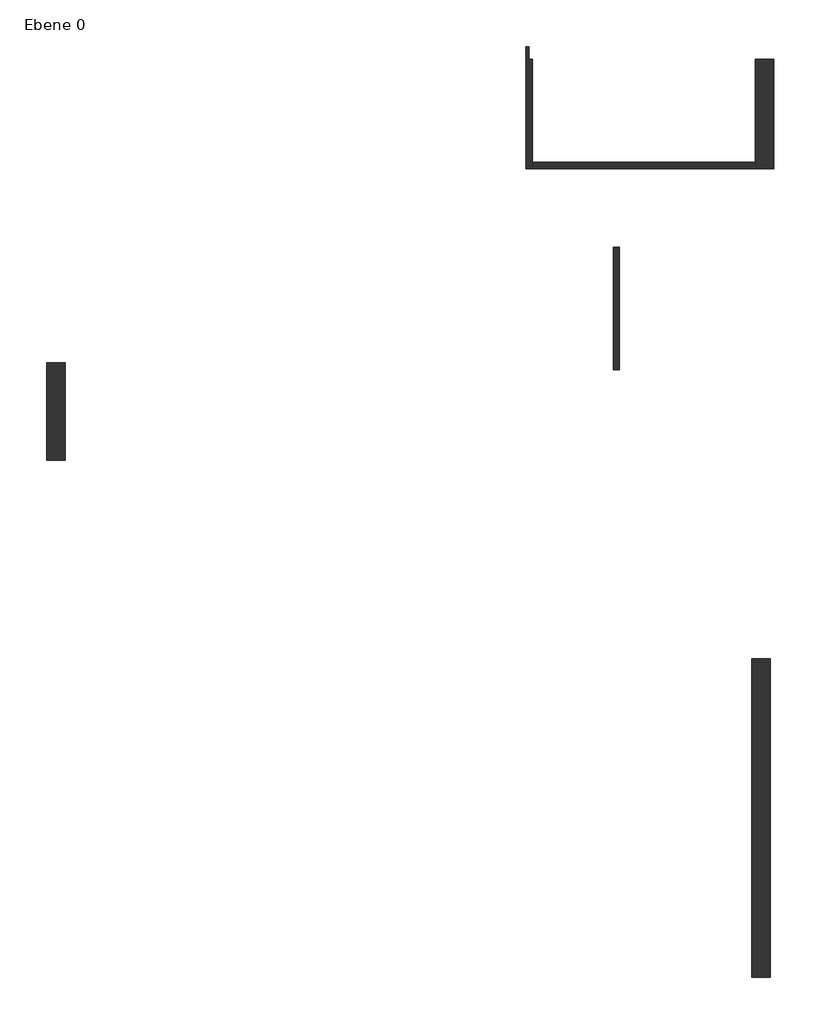
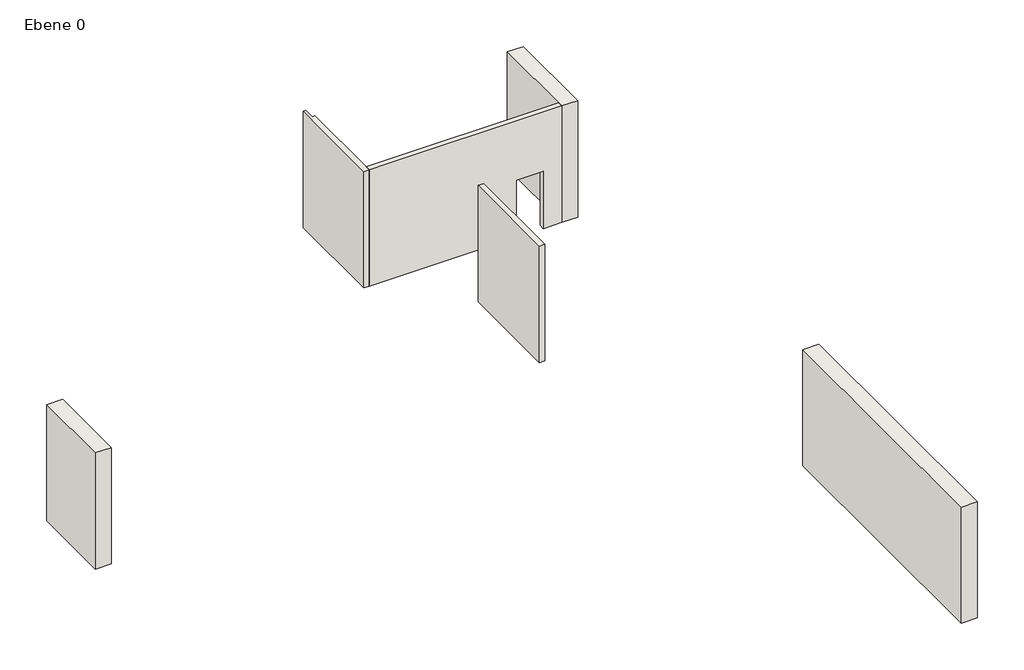
# One storey: 6 walls.
"""IFC4 building model written with IfcOpenShell, lengths in millimetres."""

import ifcopenshell
import ifcopenshell.guid

model = None  # the IFC model being written
_history = None  # IfcOwnerHistory: only IFC2X3 demands one
_inside = {}  # id of a spatial element -> (the spatial element, [elements in it])
_under = {}  # id of a project, library or spatial element -> (it, [spatial elements below it])
_declared = {}  # id of a project -> (the project, [libraries it declares])
_typed = {}  # id of a type object -> (the type object, [elements of that type])
_made_of = {}  # id of a material, layer set ... -> (it, [elements and type objects made of it])


def new_model(schema):
    """Start an empty IFC model of exactly this schema.

    Asked for "IFC4X3", IfcOpenShell would pick the latest addendum, in which some entities
    have other attributes; the version numbers below select the first issue.
    IFC2X3 requires an IfcOwnerHistory on every rooted entity: one is made here for all.
    """
    global model, _history
    if schema == "IFC4X3":
        model = ifcopenshell.file(schema_version=(4, 3, 0, 0))
    else:
        model = ifcopenshell.file(schema=schema)
    _inside.clear()
    _under.clear()
    _declared.clear()
    _typed.clear()
    _made_of.clear()
    _history = None
    if model.schema == "IFC2X3":
        org = make("IfcOrganization", Name="unknown")
        user = make(
            "IfcPersonAndOrganization",
            ThePerson=make("IfcPerson", FamilyName="unknown"),
            TheOrganization=org,
        )
        app = make(
            "IfcApplication",
            ApplicationDeveloper=org,
            Version="unknown",
            ApplicationFullName="unknown",
            ApplicationIdentifier="unknown",
        )
        _history = make(
            "IfcOwnerHistory",
            OwningUser=user,
            OwningApplication=app,
            ChangeAction="ADDED",
            CreationDate=0,
        )
    return model


def make(cls, **values):
    """One entity of the class cls with the attributes given. An attribute that is None is left unset."""
    return model.create_entity(
        cls, **{name: value for name, value in values.items() if value is not None}
    )


def rooted(cls, **values):
    """An entity with a GlobalId (a new one), such as an element, a storey or a relation."""
    return make(cls, GlobalId=ifcopenshell.guid.new(), OwnerHistory=_history, **values)


def si_unit(unit_type, name, prefix=None):
    """IfcSIUnit, for example si_unit("LENGTHUNIT", "METRE", prefix="MILLI")."""
    return make("IfcSIUnit", UnitType=unit_type, Prefix=prefix, Name=name)


def assignment(units):
    """IfcUnitAssignment: the units of a project."""
    return None if units is None else make("IfcUnitAssignment", Units=units)


def point(xyz):
    """IfcCartesianPoint."""
    return None if xyz is None else make("IfcCartesianPoint", Coordinates=xyz)


def direction(xyz):
    """IfcDirection."""
    return None if xyz is None else make("IfcDirection", DirectionRatios=xyz)


def frame(location, z_axis=None, x_axis=None):
    """IfcAxis2Placement3D, a coordinate frame: its origin and axes. An axis left out is left unset."""
    return make(
        "IfcAxis2Placement3D",
        Location=point(location),
        Axis=direction(z_axis),
        RefDirection=direction(x_axis),
    )


def origin():
    """The frame at (0, 0, 0) with its axes left unset."""
    return frame((0.0, 0.0, 0.0))


def place(relative_to, where):
    """IfcLocalPlacement: puts the frame where relative to a parent placement (None: the world)."""
    return make(
        "IfcLocalPlacement", PlacementRelTo=relative_to, RelativePlacement=where
    )


def context(
    kind, dimensions, precision=None, world=None, true_north=None, identifier=None
):
    """IfcGeometricRepresentationContext, for example the 3D "Model" context."""
    return make(
        "IfcGeometricRepresentationContext",
        ContextIdentifier=identifier,
        ContextType=kind,
        CoordinateSpaceDimension=dimensions,
        Precision=precision,
        WorldCoordinateSystem=world,
        TrueNorth=true_north,
    )


def project(units=None, contexts=None):
    """IfcProject with its units and contexts."""
    return rooted(
        "IfcProject",
        Name="project",
        RepresentationContexts=contexts,
        UnitsInContext=assignment(units),
    )


def spatial(cls, under=None, at=None, **own):
    """A site, building, storey or space (cls), placed at a placement, below another one or the project."""
    s = rooted(cls, ObjectPlacement=at, **own)
    if under is not None:
        _under.setdefault(under.id(), (under, []))[1].append(s)
    return s


def polyline(points):
    """IfcPolyline through the points."""
    return make("IfcPolyline", Points=[point(p) for p in points])


def outline(outer, holes=None, kind="AREA"):
    """IfcArbitraryClosedProfileDef: a profile drawn as a closed curve; with holes, ...WithVoids."""
    if holes is None:
        return make("IfcArbitraryClosedProfileDef", ProfileType=kind, OuterCurve=outer)
    return make(
        "IfcArbitraryProfileDefWithVoids",
        ProfileType=kind,
        OuterCurve=outer,
        InnerCurves=holes,
    )


def extrude(swept, where, along, depth):
    """IfcExtrudedAreaSolid: the profile swept, set in the frame where, extruded along a direction by depth."""
    return make(
        "IfcExtrudedAreaSolid",
        SweptArea=swept,
        Position=where,
        ExtrudedDirection=direction(along),
        Depth=depth,
    )


def faces_of(points, faces, orient=None, outer=None):
    """IfcFace entities. A face is a list of loops; a loop is a list of indices into points, from 0.

    orient and outer hold one flag for each loop. By default every Orientation is true, the
    first loop of a face is its IfcFaceOuterBound and the others are IfcFaceBound.
    """
    made = []
    for i, loops in enumerate(faces):
        bounds = []
        for j, loop in enumerate(loops):
            is_outer = j == 0 if outer is None else outer[i][j]
            bounds.append(
                make(
                    "IfcFaceOuterBound" if is_outer else "IfcFaceBound",
                    Bound=make("IfcPolyLoop", Polygon=[points[k] for k in loop]),
                    Orientation=True if orient is None else orient[i][j],
                )
            )
        made.append(make("IfcFace", Bounds=bounds))
    return made


def faceted_brep(points, faces, orient=None, outer=None, voids=None):
    """IfcFacetedBrep: a solid bounded by flat faces; with voids (closed shells), ...WithVoids."""
    shared = [point(p) for p in points]
    hull = make("IfcClosedShell", CfsFaces=faces_of(shared, faces, orient, outer))
    if voids is None:
        return make("IfcFacetedBrep", Outer=hull)
    return make(
        "IfcFacetedBrepWithVoids",
        Outer=hull,
        Voids=[
            make(cls, CfsFaces=faces_of(shared, fs, o, b)) for cls, fs, o, b in voids
        ],
    )


def shape(context_of_items, identifier, shape_type, items):
    """IfcShapeRepresentation: the items that make up one representation, for example the "Body"."""
    return make(
        "IfcShapeRepresentation",
        ContextOfItems=context_of_items,
        RepresentationIdentifier=identifier,
        RepresentationType=shape_type,
        Items=items,
    )


def made_of(thing, what):
    """Note that an element or type object is made of a material, layer set ...; save() writes the relation."""
    if what is not None:
        _made_of.setdefault(what.id(), (what, []))[1].append(thing)
    return thing


def element(
    cls,
    number,
    at=None,
    inside=None,
    cuts=None,
    type_object=None,
    material=None,
    context=None,
    identifier="Body",
    shape_type=None,
    held_by="IfcProductDefinitionShape",
    body=None,
    shapes=None,
    **own,
):
    """One element of the class cls, such as IfcWall. Its Tag is "e" and its number.

    at: its placement. inside: the storey or other place that contains it. cuts: it is an
    opening in that element (IfcRelVoidsElement). A single representation is given by context,
    identifier, shape_type and body (its items); several are given by shapes. held_by: the class
    of the entity that holds the representations. save() writes the other relations.
    """
    e = rooted(cls, Tag="e%d" % number, ObjectPlacement=at, **own)
    if body is not None:
        shapes = [shape(context, identifier, shape_type, body)]
    if shapes is not None:
        e.Representation = make(held_by, Representations=shapes)
    if inside is not None:
        _inside.setdefault(inside.id(), (inside, []))[1].append(e)
    if cuts is not None:
        rooted(
            "IfcRelVoidsElement", RelatingBuildingElement=cuts, RelatedOpeningElement=e
        )
    if type_object is not None:
        _typed.setdefault(type_object.id(), (type_object, []))[1].append(e)
    return made_of(e, material)


def aggregate(whole, parts):
    """IfcRelAggregates: a whole, such as a stair, and the parts it consists of."""
    return rooted("IfcRelAggregates", RelatingObject=whole, RelatedObjects=parts)


def save(model, path):
    """Write the relations noted so far, then the file.

    IfcRelAggregates (storeys below a building ...), IfcRelContainedInSpatialStructure (elements
    in a storey), IfcRelDefinesByType, IfcRelAssociatesMaterial and IfcRelDeclares: one each for
    every whole, place, type object, material and project.
    """
    for whole, parts in _under.values():
        aggregate(whole, parts)
    for where, things in _inside.values():
        rooted(
            "IfcRelContainedInSpatialStructure",
            RelatedElements=things,
            RelatingStructure=where,
        )
    for kind, things in _typed.values():
        rooted("IfcRelDefinesByType", RelatedObjects=things, RelatingType=kind)
    for what, things in _made_of.values():
        rooted("IfcRelAssociatesMaterial", RelatedObjects=things, RelatingMaterial=what)
    for by, libraries in _declared.values():
        rooted("IfcRelDeclares", RelatingContext=by, RelatedDefinitions=libraries)
    model.write(path)


model = new_model("IFC4")

# Units and contexts
model_context = context("Model", 3, world=origin())
ifc_project = project(units=[si_unit("LENGTHUNIT", "METRE", prefix="MILLI")], contexts=[model_context])

# Site, building, storey
site = spatial("IfcSite", under=ifc_project)
building = spatial("IfcBuilding", under=site)
storey = spatial("IfcBuildingStorey", under=building, Name="Ebene 0", Elevation=0.0)

# Walls
placement = place(None, origin())
element("IfcWall", 1, ObjectType="STB 20.0", at=placement, inside=storey, context=model_context, shape_type="Brep", body=[
    faceted_brep([(5655.3173257, 15397.2389222, -1570.0), (5655.3173257, 11462.2122385, -1570.0), (5655.3173257, 11462.2122385, 3030.0), (5655.3173257, 15397.2389222, 3030.0), (5855.3173257, 14985.0055214, -1570.0), (5855.3173257, 14985.0055214, 3030.0), (5855.3173257, 11662.2122385, 3030.0), (5855.3173257, 11462.2122385, 3030.0), (5855.3173257, 11462.2122385, -1570.0), (5855.3173257, 11662.2122385, -1570.0), (5755.3173257, 15397.2389222, -1570.0), (5755.3173257, 14985.0055214, -1570.0), (5755.3173257, 14985.0055214, 3030.0), (5755.3173257, 15397.2389222, 3030.0)], [[[0, 1, 2, 3]], [[4, 5, 6, 7, 8, 9]], [[1, 0, 10, 11, 4, 9, 8]], [[3, 2, 7, 6, 5, 12, 13]], [[0, 3, 13, 10]], [[13, 12, 11, 10]], [[12, 5, 4, 11]], [[2, 1, 8, 7]]]),
])
element("IfcWall", 2, ObjectType="STB 20.0", at=placement, inside=storey, context=model_context, shape_type="SweptSolid", body=[
    extrude(outline(polyline([(3030.0, 13055.3173257), (3030.0, 5855.3173257), (-1570.0, 5855.3173257), (-1570.0, 11355.3173257), (690.0, 11355.3173257), (690.0, 12355.3173257), (-1570.0, 12355.3173257), (-1570.0, 13055.3173257), (3030.0, 13055.3173257)])), frame((0.0, 11462.2122385, 0.0), z_axis=(0.0, 1.0, 0.0), x_axis=(0.0, 0.0, 1.0)), (0.0, 0.0, 1.0), 200.0),
])
element("IfcWall", 3, ObjectType="STB 20.0", at=placement, inside=storey, context=model_context, shape_type="Brep", body=[
    faceted_brep([(8468.8165485, 8930.3849854, -1570.0), (8468.8165485, 4972.602282, -1570.0), (8468.8165485, 4972.602282, 3030.0), (8468.8165485, 8930.3849854, 3030.0), (8668.8165485, 8930.3849854, -1570.0), (8668.8165485, 8930.3849854, 3030.0), (8668.8165485, 5172.602282, 3030.0), (8668.8165485, 4972.602282, 3030.0), (8668.8165485, 4972.602282, -1570.0)], [[[0, 1, 2, 3]], [[4, 5, 6, 7, 8]], [[1, 0, 4, 8]], [[3, 2, 7, 6, 5]], [[0, 3, 5, 4]], [[2, 1, 8, 7]]]),
])
element("IfcWall", 4, ObjectType="STB 48 schwarz", at=placement, inside=storey, context=model_context, shape_type="Brep", body=[
    faceted_brep([(13533.9896827, -14619.7385411, -1554.3161242), (13533.9896827, -4351.0115596, -1554.3161242), (13533.9896827, -4351.0115596, 3031.4905816), (13533.9896827, -14619.7385411, 3031.4905816), (13533.9896827, -14619.7385411, 3030.0), (12933.9896827, -14619.7385411, -1554.3161242), (12933.9896827, -14619.7385411, 3031.4905816), (12933.9896827, -4351.0115596, 3031.4905816), (12933.9896827, -4351.0115596, 3030.0), (12933.9896827, -4351.0115596, -1554.3161242)], [[[0, 1, 2, 3, 4]], [[5, 6, 7, 8, 9]], [[1, 0, 5, 9]], [[3, 2, 7, 6]], [[2, 1, 9, 8, 7]], [[0, 4, 3, 6, 5]]]),
])
element("IfcWall", 5, ObjectType="STB 48.0 WD 12.0", at=placement, inside=storey, context=model_context, shape_type="Brep", body=[
    faceted_brep([(13055.3173257, 14985.0055214, -1574.7000647), (13055.3173257, 11462.2122385, -1574.7000647), (13055.3173257, 11462.2122385, -1570.0), (13055.3173257, 11462.2122385, 3030.0), (13055.3173257, 11462.2122385, 3031.5985486), (13055.3173257, 14985.0055214, 3031.5985486), (13655.3173257, 14985.0055214, -1574.7000647), (13655.3173257, 14985.0055214, -1570.0), (13655.3173257, 14985.0055214, 3030.0), (13655.3173257, 14985.0055214, 3031.5985486), (13655.3173257, 11462.2122385, 3031.5985486), (13655.3173257, 11462.2122385, -1574.7000647)], [[[0, 1, 2, 3, 4, 5]], [[6, 7, 8, 9, 10, 11]], [[1, 0, 6, 11]], [[5, 4, 10, 9]], [[0, 5, 9, 8, 7, 6]], [[4, 3, 2, 1, 11, 10]]]),
])
element("IfcWall", 6, ObjectType="STB 48.0 WD 12.0", at=placement, inside=storey, context=model_context, shape_type="SweptSolid", body=[
    extrude(outline(polyline([(-9817.3070453, 2054.3111004), (-9817.3070453, 5207.5084574), (-9217.3070453, 5207.5084574), (-9217.3070453, 2054.3111004), (-9817.3070453, 2054.3111004)])), frame((0.0, 0.0, -1562.4482239), z_axis=(0.0, 0.0, 1.0), x_axis=(1.0, 0.0, 0.0)), (0.0, 0.0, 1.0), 4592.8837826),
])

save(model, "model.ifc")

# Revit data of these elements
# Type "STB 20.0"
#   Type Comments = "Stahlbeton"
#   Description = "Stahlbeton 20.0"
#   Layers, outside or top first: 0.200 m "Stahlbeton - Ortbeton" (function 1)
# Type "STB 48 schwarz"
#   Type Comments = "Stahlbeton mit Wärmedämmung"
#   Description = "Stahlbeton 25.0, Wärmedämmung 12.0 cm"
#   Layers, outside or top first: 0.120 m "Wärmedämmung - hart" (function 3); 0.470 m "Stahlbeton - Ortbeton" (function 1); 0.010 m "Kunststoff - Grau" (function 1)
# Type "STB 48.0 WD 12.0"
#   Type Comments = "Stahlbeton mit Wärmedämmung"
#   Description = "Stahlbeton 25.0, Wärmedämmung 12.0 cm"
#   Layers, outside or top first: 0.120 m "Wärmedämmung - hart" (function 3); 0.480 m "Stahlbeton - Ortbeton" (function 1)
# Elements 1, 2, 3 (IfcWall, "STB 20.0")
#   Comments = ""
#   built-in parameter 1001111 = -1.570 m
#   Top Offset = 0.000 m
#   Base Offset = -1.570 m
#   wall height = 4.600 m
#   Phase Created = Phase 1
#   Base Constraint = Ebene 0
#   Top Constraint = UK Decke EG
#   Materials on its faces: "Stahlbeton - Ortbeton"
# Element 4 (IfcWall, "STB 48 schwarz")
#   Comments = ""
#   built-in parameter 1001111 = -1.554316 m
#   Top Offset = 3.031491 m
#   Base Offset = -1.554316 m
#   wall height = 4.585807 m
#   Phase Created = Phase 1
#   Base Constraint = Ebene 0
#   Top Constraint = Ebene 0
#   Materials on its faces: "Vorgabe - Wand", "Wärmedämmung - hart", "Kunststoff - Grau", "Stahlbeton - Sichtbeton (1)"
# Element 5 (IfcWall, "STB 48.0 WD 12.0")
#   Comments = ""
#   built-in parameter 1001111 = -1.5747 m
#   Top Offset = 3.031599 m
#   Base Offset = -1.5747 m
#   wall height = 4.606299 m
#   Phase Created = Phase 1
#   Base Constraint = Ebene 0
#   Top Constraint = Ebene 0
#   Materials on its faces: "Vorgabe - Wand", "Stahlbeton - Ortbeton", "Wärmedämmung - hart"
# Element 6 (IfcWall, "STB 48.0 WD 12.0")
#   Comments = ""
#   built-in parameter 1001111 = -1.562448 m
#   Top Offset = 3.030436 m
#   Base Offset = -1.562448 m
#   wall height = 4.592884 m
#   Phase Created = Phase 1
#   Base Constraint = Ebene 0
#   Top Constraint = Ebene 0
#   Materials on its faces: "Vorgabe - Wand", "Stahlbeton - Ortbeton", "Wärmedämmung - hart", "Stahlbeton - Sichtbeton (1)", "Decke - Gipskarton"
# Materials
#   "Stahlbeton - Ortbeton": class "Beton", colour RGB 247 247 247, transparency 0, Cost = 0
#   "Wärmedämmung - hart": class "Stuck", colour RGB 255 255 255, transparency 0, Description = "Äußere Oberfläche", Cost = 0
#   "Kunststoff - Grau": class "Kunststoff", colour RGB 0 0 0, transparency 0, Cost = 0
#   "Vorgabe - Wand": class "Stuck", colour RGB 128 128 128, transparency 0, Description = "Äußere Oberfläche", Cost = 0
#   "Stahlbeton - Sichtbeton (1)": class "Beton", colour RGB 192 192 192, transparency 0, Cost = 0
#   "Decke - Gipskarton": class "Trockenbauwand", colour RGB 255 255 255, transparency 0, Cost = 0
